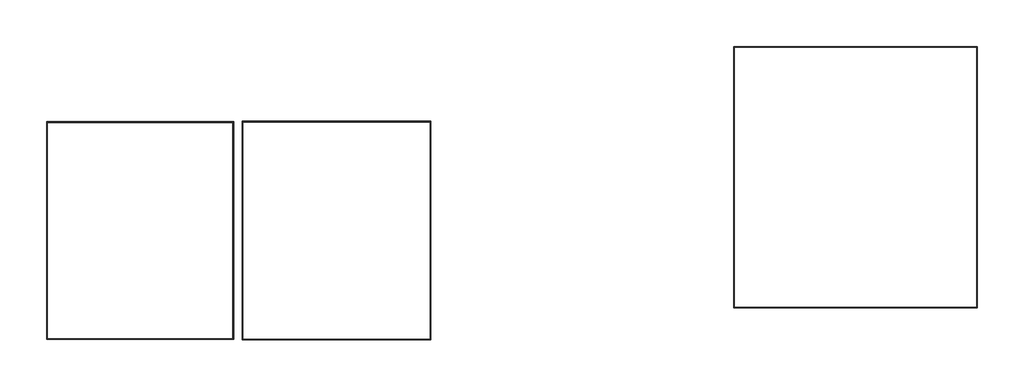
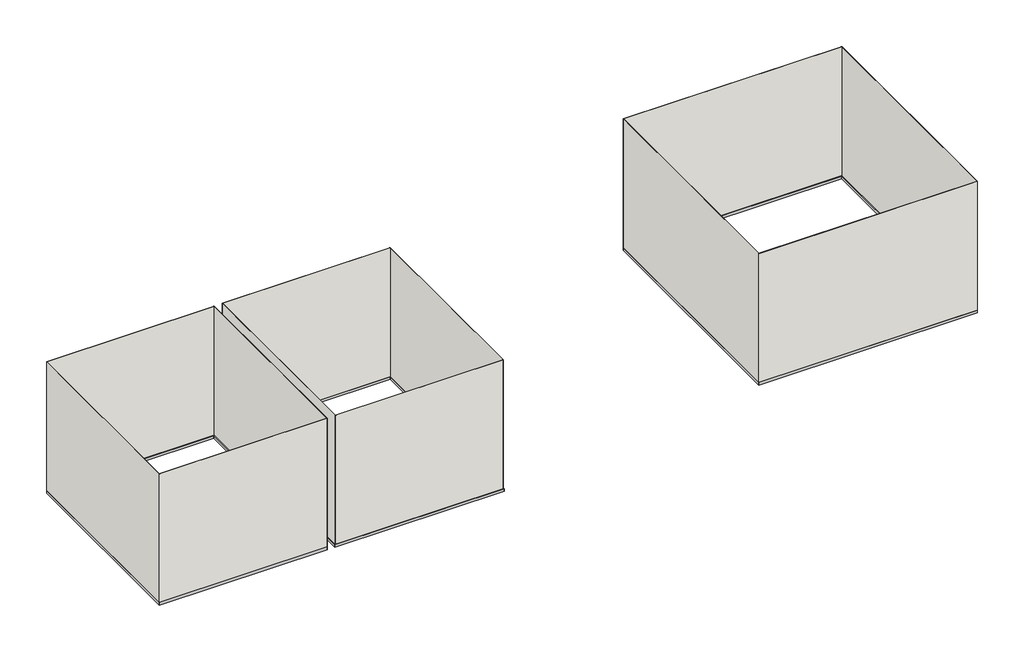
# Not in any storey: 12 proxies, 12 walls.
"""IFC4 building model written with IfcOpenShell, lengths in millimetres."""

from ifc_helpers import new_model, si_unit, frame, origin, place, context, project, spatial, polyline, outline, extrude, faceted_brep, element, save

model = new_model("IFC4")

# Units and contexts
model_context = context("Model", 3, world=origin())
ifc_project = project(units=[si_unit("LENGTHUNIT", "METRE", prefix="MILLI")], contexts=[model_context])

# Site, building
site = spatial("IfcSite", under=ifc_project)
building = spatial("IfcBuilding", under=site)

# Proxies
placement = place(None, origin())
element("IfcBuildingElementProxy", 1, Name="Wall Sweeps", at=placement, inside=building, context=model_context, shape_type="SweptSolid", body=[
    extrude(outline(polyline([(6040.0722622, 436.7286004), (6028.0722622, 448.7286004), (9910.0722622, 448.7286004), (9898.0722622, 436.7286004), (6040.0722622, 436.7286004)])), frame((0.0, 0.0, 12090.0), z_axis=(0.0, 0.0, 1.0), x_axis=(1.0, 0.0, 0.0)), (0.0, 0.0, 1.0), 50.0),
])
element("IfcBuildingElementProxy", 2, Name="Wall Sweeps", at=placement, inside=building, context=model_context, shape_type="Brep", body=[
    faceted_brep([(9898.0722622, 436.7286004, 12090.0), (9898.0722622, 436.7286004, 12140.0), (9910.0722622, 448.7286004, 12140.0), (9910.0722622, 448.7286004, 12090.0), (9898.0722622, -3708.7713618, 12090.0), (9910.0722622, -3720.7713618, 12090.0), (9910.0722622, -3720.7713618, 12140.0), (9898.0722622, -3708.7713618, 12140.0), (9910.0722622, 446.7286004, 12140.0)], [[[0, 1, 2, 3]], [[4, 5, 6, 7]], [[1, 0, 4, 7]], [[2, 1, 7, 6, 8]], [[3, 2, 8, 6, 5]], [[0, 3, 5, 4]]]),
])
element("IfcBuildingElementProxy", 3, Name="Wall Sweeps", at=placement, inside=building, context=model_context, shape_type="Brep", body=[
    faceted_brep([(9898.0722622, -3708.7713618, 12090.0), (9898.0722622, -3708.7713618, 12140.0), (9910.0722622, -3720.7713618, 12140.0), (9910.0722622, -3720.7713618, 12090.0), (6040.0722622, -3708.7713618, 12090.0), (6028.0722622, -3720.7713618, 12090.0), (6028.0722622, -3720.7713618, 12140.0), (6040.0722622, -3708.7713618, 12140.0), (9908.0722622, -3720.7713618, 12140.0)], [[[0, 1, 2, 3]], [[4, 5, 6, 7]], [[1, 0, 4, 7]], [[2, 1, 7, 6, 8]], [[3, 2, 8, 6, 5]], [[0, 3, 5, 4]]]),
])
element("IfcBuildingElementProxy", 4, Name="Wall Sweeps", at=placement, inside=building, context=model_context, shape_type="Brep", body=[
    faceted_brep([(6040.0722622, -3708.7713618, 12090.0), (6040.0722622, -3708.7713618, 12140.0), (6028.0722622, -3720.7713618, 12140.0), (6028.0722622, -3720.7713618, 12090.0), (6040.0722622, 436.7286004, 12090.0), (6028.0722622, 448.7286004, 12090.0), (6028.0722622, 448.7286004, 12140.0), (6040.0722622, 436.7286004, 12140.0), (6028.0722622, 446.7286004, 12140.0), (6028.0722622, -3718.7713618, 12140.0)], [[[0, 1, 2, 3]], [[4, 5, 6, 7]], [[1, 0, 4, 7]], [[2, 1, 7, 6, 8, 9]], [[3, 2, 9, 8, 6, 5]], [[0, 3, 5, 4]]]),
])
element("IfcBuildingElementProxy", 5, Name="Wall Sweeps", at=placement, inside=building, context=model_context, shape_type="SweptSolid", body=[
    extrude(outline(polyline([(-1799.4277378, -4230.7713618), (-1787.4277378, -4218.7713618), (1195.5722622, -4218.7713618), (1207.5722622, -4230.7713618), (-1799.4277378, -4230.7713618)])), frame((0.0, 0.0, 12090.0), z_axis=(0.0, 0.0, 1.0), x_axis=(1.0, 0.0, 0.0)), (0.0, 0.0, 1.0), 50.0),
])
element("IfcBuildingElementProxy", 6, Name="Wall Sweeps", at=placement, inside=building, context=model_context, shape_type="SweptSolid", body=[
    extrude(outline(polyline([(1207.5722622, -4230.7713618), (1195.5722622, -4218.7713618), (1195.5722622, -753.2713618), (1207.5722622, -741.2713618), (1207.5722622, -4230.7713618)])), frame((0.0, 0.0, 12090.0), z_axis=(0.0, 0.0, 1.0), x_axis=(1.0, 0.0, 0.0)), (0.0, 0.0, 1.0), 50.0),
])
element("IfcBuildingElementProxy", 7, Name="Wall Sweeps", at=placement, inside=building, context=model_context, shape_type="SweptSolid", body=[
    extrude(outline(polyline([(1207.5722622, -741.2713618), (1195.5722622, -753.2713618), (-1787.4277378, -753.2713618), (-1799.4277378, -741.2713618), (1207.5722622, -741.2713618)])), frame((0.0, 0.0, 12090.0), z_axis=(0.0, 0.0, 1.0), x_axis=(1.0, 0.0, 0.0)), (0.0, 0.0, 1.0), 50.0),
])
element("IfcBuildingElementProxy", 8, Name="Wall Sweeps", at=placement, inside=building, context=model_context, shape_type="SweptSolid", body=[
    extrude(outline(polyline([(-1799.4277378, -741.2713618), (-1787.4277378, -753.2713618), (-1787.4277378, -4218.7713618), (-1799.4277378, -4230.7713618), (-1799.4277378, -741.2713618)])), frame((0.0, 0.0, 12090.0), z_axis=(0.0, 0.0, 1.0), x_axis=(1.0, 0.0, 0.0)), (0.0, 0.0, 1.0), 50.0),
])
element("IfcBuildingElementProxy", 9, Name="Wall Sweeps", at=placement, inside=building, context=model_context, shape_type="SweptSolid", body=[
    extrude(outline(polyline([(-4899.9277378, -763.2713996), (-4911.9277378, -751.2713996), (-1932.4277378, -751.2713996), (-1944.4277378, -763.2713996), (-4899.9277378, -763.2713996)])), frame((0.0, 0.0, 12090.0), z_axis=(0.0, 0.0, 1.0), x_axis=(1.0, 0.0, 0.0)), (0.0, 0.0, 1.0), 50.0),
])
element("IfcBuildingElementProxy", 10, Name="Wall Sweeps", at=placement, inside=building, context=model_context, shape_type="Brep", body=[
    faceted_brep([(-1944.4277378, -763.2713996, 12090.0), (-1944.4277378, -763.2713996, 12140.0), (-1932.4277378, -751.2713996, 12140.0), (-1932.4277378, -751.2713996, 12090.0), (-1944.4277378, -4208.7713618, 12090.0), (-1932.4277378, -4220.7713618, 12090.0), (-1932.4277378, -4220.7713618, 12140.0), (-1944.4277378, -4208.7713618, 12140.0), (-1932.4277378, -753.2713996, 12140.0)], [[[0, 1, 2, 3]], [[4, 5, 6, 7]], [[1, 0, 4, 7]], [[2, 1, 7, 6, 8]], [[3, 2, 8, 6, 5]], [[0, 3, 5, 4]]]),
])
element("IfcBuildingElementProxy", 11, Name="Wall Sweeps", at=placement, inside=building, context=model_context, shape_type="Brep", body=[
    faceted_brep([(-1944.4277378, -4208.7713618, 12090.0), (-1944.4277378, -4208.7713618, 12140.0), (-1932.4277378, -4220.7713618, 12140.0), (-1932.4277378, -4220.7713618, 12090.0), (-4899.9277378, -4208.7713618, 12090.0), (-4911.9277378, -4220.7713618, 12090.0), (-4911.9277378, -4220.7713618, 12140.0), (-4899.9277378, -4208.7713618, 12140.0), (-1934.4277378, -4220.7713618, 12140.0)], [[[0, 1, 2, 3]], [[4, 5, 6, 7]], [[1, 0, 4, 7]], [[2, 1, 7, 6, 8]], [[3, 2, 8, 6, 5]], [[0, 3, 5, 4]]]),
])
element("IfcBuildingElementProxy", 12, Name="Wall Sweeps", at=placement, inside=building, context=model_context, shape_type="Brep", body=[
    faceted_brep([(-4899.9277378, -4208.7713618, 12090.0), (-4899.9277378, -4208.7713618, 12140.0), (-4911.9277378, -4220.7713618, 12140.0), (-4911.9277378, -4220.7713618, 12090.0), (-4899.9277378, -763.2713996, 12090.0), (-4911.9277378, -751.2713996, 12090.0), (-4911.9277378, -751.2713996, 12140.0), (-4899.9277378, -763.2713996, 12140.0), (-4911.9277378, -753.2713996, 12140.0), (-4911.9277378, -4218.7713618, 12140.0)], [[[0, 1, 2, 3]], [[4, 5, 6, 7]], [[1, 0, 4, 7]], [[2, 1, 7, 6, 8, 9]], [[3, 2, 9, 8, 6, 5]], [[0, 3, 5, 4]]]),
])

# Walls
element("IfcWall", 13, ObjectType="W_D=벽지/거실+걸레받이#", at=placement, inside=building, context=model_context, shape_type="Brep", body=[
    faceted_brep([(9910.0722622, 446.7286004, 14560.0), (9908.0722622, 446.7286004, 14560.0), (6030.0722622, 446.7286004, 14560.0), (6028.0722622, 446.7286004, 14560.0), (6028.0722622, 446.7286004, 12140.0), (6030.0722622, 446.7286004, 12140.0), (9908.0722622, 446.7286004, 12140.0), (9910.0722622, 446.7286004, 12140.0), (6028.0722622, 448.7286004, 14560.0), (9910.0722622, 448.7286004, 14560.0), (9910.0722622, 448.7286004, 12140.0), (6028.0722622, 448.7286004, 12140.0)], [[[0, 1, 2, 3, 4, 5, 6, 7]], [[8, 9, 10, 11]], [[3, 2, 1, 0, 9, 8]], [[9, 0, 7, 10]], [[3, 8, 11, 4]], [[7, 6, 5, 4, 11, 10]]]),
])
element("IfcWall", 14, ObjectType="W_D=벽지/거실+걸레받이#", at=placement, inside=building, context=model_context, shape_type="Brep", body=[
    faceted_brep([(9908.0722622, -3720.7713618, 14560.0), (9908.0722622, -3718.7713618, 14560.0), (9908.0722622, 446.7286004, 14560.0), (9908.0722622, 446.7286004, 12140.0), (9908.0722622, -3718.7713618, 12140.0), (9908.0722622, -3720.7713618, 12140.0), (9910.0722622, 446.7286004, 14560.0), (9910.0722622, -3720.7713618, 14560.0), (9910.0722622, -3720.7713618, 12140.0), (9910.0722622, 446.7286004, 12140.0)], [[[0, 1, 2, 3, 4, 5]], [[6, 7, 8, 9]], [[2, 1, 0, 7, 6]], [[7, 0, 5, 8]], [[2, 6, 9, 3]], [[5, 4, 3, 9, 8]]]),
])
element("IfcWall", 15, ObjectType="W_D=벽지/거실+걸레받이#", at=placement, inside=building, context=model_context, shape_type="Brep", body=[
    faceted_brep([(6028.0722622, -3718.7713618, 14560.0), (6030.0722622, -3718.7713618, 14560.0), (9908.0722622, -3718.7713618, 14560.0), (9908.0722622, -3718.7713618, 12140.0), (6030.0722622, -3718.7713618, 12140.0), (6028.0722622, -3718.7713618, 12140.0), (9908.0722622, -3720.7713618, 14560.0), (6028.0722622, -3720.7713618, 14560.0), (6028.0722622, -3720.7713618, 12140.0), (9908.0722622, -3720.7713618, 12140.0)], [[[0, 1, 2, 3, 4, 5]], [[6, 7, 8, 9]], [[2, 1, 0, 7, 6]], [[7, 0, 5, 8]], [[2, 6, 9, 3]], [[5, 4, 3, 9, 8]]]),
])
element("IfcWall", 16, ObjectType="W_D=벽지/거실+걸레받이#", at=placement, inside=building, context=model_context, shape_type="SweptSolid", body=[
    extrude(outline(polyline([(6030.0722622, 446.7286004), (6030.0722622, -3718.7713618), (6028.0722622, -3718.7713618), (6028.0722622, 446.7286004), (6030.0722622, 446.7286004)])), frame((0.0, 0.0, 12140.0), z_axis=(0.0, 0.0, 1.0), x_axis=(1.0, 0.0, 0.0)), (0.0, 0.0, 1.0), 2420.0),
])
element("IfcWall", 17, ObjectType="W_D=벽지/거실+걸레받이#", at=placement, inside=building, context=model_context, shape_type="Brep", body=[
    faceted_brep([(1197.5722622, -4220.7713618, 14560.0), (-1789.4277378, -4220.7713618, 14560.0), (-1789.4277378, -4220.7713618, 12140.0), (1197.5722622, -4220.7713618, 12140.0), (-1789.4277378, -4218.7713618, 14560.0), (-1787.4277378, -4218.7713618, 14560.0), (1195.5722622, -4218.7713618, 14560.0), (1197.5722622, -4218.7713618, 14560.0), (1197.5722622, -4218.7713618, 12140.0), (1195.5722622, -4218.7713618, 12140.0), (-1787.4277378, -4218.7713618, 12140.0), (-1789.4277378, -4218.7713618, 12140.0)], [[[0, 1, 2, 3]], [[4, 5, 6, 7, 8, 9, 10, 11]], [[1, 0, 7, 6, 5, 4]], [[7, 0, 3, 8]], [[1, 4, 11, 2]], [[3, 2, 11, 10, 9, 8]]]),
])
element("IfcWall", 18, ObjectType="W_D=벽지/거실+걸레받이#", at=placement, inside=building, context=model_context, shape_type="Brep", body=[
    faceted_brep([(1197.5722622, -751.2713618, 14560.0), (1197.5722622, -4218.7713618, 14560.0), (1197.5722622, -4218.7713618, 12140.0), (1197.5722622, -751.2713618, 12140.0), (1195.5722622, -4218.7713618, 14560.0), (1195.5722622, -753.2713618, 14560.0), (1195.5722622, -751.2713618, 14560.0), (1195.5722622, -751.2713618, 12140.0), (1195.5722622, -753.2713618, 12140.0), (1195.5722622, -4218.7713618, 12140.0)], [[[0, 1, 2, 3]], [[4, 5, 6, 7, 8, 9]], [[1, 0, 6, 5, 4]], [[6, 0, 3, 7]], [[1, 4, 9, 2]], [[3, 2, 9, 8, 7]]]),
])
element("IfcWall", 19, ObjectType="W_D=벽지/거실+걸레받이#", at=placement, inside=building, context=model_context, shape_type="Brep", body=[
    faceted_brep([(-1789.4277378, -751.2713618, 14560.0), (1195.5722622, -751.2713618, 14560.0), (1195.5722622, -751.2713618, 12140.0), (-1789.4277378, -751.2713618, 12140.0), (1195.5722622, -753.2713618, 14560.0), (-1787.4277378, -753.2713618, 14560.0), (-1789.4277378, -753.2713618, 14560.0), (-1789.4277378, -753.2713618, 12140.0), (-1787.4277378, -753.2713618, 12140.0), (1195.5722622, -753.2713618, 12140.0)], [[[0, 1, 2, 3]], [[4, 5, 6, 7, 8, 9]], [[1, 0, 6, 5, 4]], [[6, 0, 3, 7]], [[1, 4, 9, 2]], [[3, 2, 9, 8, 7]]]),
])
element("IfcWall", 20, ObjectType="W_D=벽지/거실+걸레받이#", at=placement, inside=building, context=model_context, shape_type="SweptSolid", body=[
    extrude(outline(polyline([(-1789.4277378, -4218.7713618), (-1789.4277378, -753.2713618), (-1787.4277378, -753.2713618), (-1787.4277378, -4218.7713618), (-1789.4277378, -4218.7713618)])), frame((0.0, 0.0, 12140.0), z_axis=(0.0, 0.0, 1.0), x_axis=(1.0, 0.0, 0.0)), (0.0, 0.0, 1.0), 2420.0),
])
element("IfcWall", 21, ObjectType="W_D=벽지/거실+걸레받이#", at=placement, inside=building, context=model_context, shape_type="Brep", body=[
    faceted_brep([(-1932.4277378, -753.2713996, 14560.0), (-1934.4277378, -753.2713996, 14560.0), (-4909.9277378, -753.2713996, 14560.0), (-4911.9277378, -753.2713996, 14560.0), (-4911.9277378, -753.2713996, 12140.0), (-4909.9277378, -753.2713996, 12140.0), (-1934.4277378, -753.2713996, 12140.0), (-1932.4277378, -753.2713996, 12140.0), (-4911.9277378, -751.2713996, 14560.0), (-1932.4277378, -751.2713996, 14560.0), (-1932.4277378, -751.2713996, 12140.0), (-4911.9277378, -751.2713996, 12140.0)], [[[0, 1, 2, 3, 4, 5, 6, 7]], [[8, 9, 10, 11]], [[3, 2, 1, 0, 9, 8]], [[9, 0, 7, 10]], [[3, 8, 11, 4]], [[7, 6, 5, 4, 11, 10]]]),
])
element("IfcWall", 22, ObjectType="W_D=벽지/거실+걸레받이#", at=placement, inside=building, context=model_context, shape_type="Brep", body=[
    faceted_brep([(-1934.4277378, -4220.7713618, 14560.0), (-1934.4277378, -4218.7713618, 14560.0), (-1934.4277378, -753.2713996, 14560.0), (-1934.4277378, -753.2713996, 12140.0), (-1934.4277378, -4218.7713618, 12140.0), (-1934.4277378, -4220.7713618, 12140.0), (-1932.4277378, -753.2713996, 14560.0), (-1932.4277378, -4220.7713618, 14560.0), (-1932.4277378, -4220.7713618, 12140.0), (-1932.4277378, -753.2713996, 12140.0)], [[[0, 1, 2, 3, 4, 5]], [[6, 7, 8, 9]], [[2, 1, 0, 7, 6]], [[7, 0, 5, 8]], [[2, 6, 9, 3]], [[5, 4, 3, 9, 8]]]),
])
element("IfcWall", 23, ObjectType="W_D=벽지/거실+걸레받이#", at=placement, inside=building, context=model_context, shape_type="Brep", body=[
    faceted_brep([(-4911.9277378, -4218.7713618, 14560.0), (-4909.9277378, -4218.7713618, 14560.0), (-1934.4277378, -4218.7713618, 14560.0), (-1934.4277378, -4218.7713618, 12140.0), (-4909.9277378, -4218.7713618, 12140.0), (-4911.9277378, -4218.7713618, 12140.0), (-1934.4277378, -4220.7713618, 14560.0), (-4911.9277378, -4220.7713618, 14560.0), (-4911.9277378, -4220.7713618, 12140.0), (-1934.4277378, -4220.7713618, 12140.0)], [[[0, 1, 2, 3, 4, 5]], [[6, 7, 8, 9]], [[2, 1, 0, 7, 6]], [[7, 0, 5, 8]], [[2, 6, 9, 3]], [[5, 4, 3, 9, 8]]]),
])
element("IfcWall", 24, ObjectType="W_D=벽지/거실+걸레받이#", at=placement, inside=building, context=model_context, shape_type="SweptSolid", body=[
    extrude(outline(polyline([(-4909.9277378, -753.2713996), (-4909.9277378, -4218.7713618), (-4911.9277378, -4218.7713618), (-4911.9277378, -753.2713996), (-4909.9277378, -753.2713996)])), frame((0.0, 0.0, 12140.0), z_axis=(0.0, 0.0, 1.0), x_axis=(1.0, 0.0, 0.0)), (0.0, 0.0, 1.0), 2420.0),
])

save(model, "model.ifc")

# Revit data of these elements
# Project information
#   Project Issue Date = "발행 날짜"
#   Project Status = "프로젝트 상태"
#   Client Name = "소유자"
#   Project Address = "주소를 여기에 입력"
#   Project Name = "프로젝트 이름"
#   Project Number = "프로젝트 번호"
#   DBIM_PRJINFO = "190232▤101▤01▤01▤▤1"
#   DBIM_ISSELECTEDHOSH = "N"
#   DBIM_STAIRS_OF_CARRIAGE = "<DBIM_STAIRS_OF_CARRIAGE>\n  <xs:schema id=\"DBIM_STAIRS_OF_CARRIAGE\" xmlns=\"\" xmlns:xs=\"http://www.w3.org/2001/XMLSchema\" xmlns:msdata=\"urn:schemas-microsoft-com:xml-msdata\">\n    <xs:element name=\"DBIM_STAIRS_OF_CARRIAGE\" msdata:IsDataSet=\"true\" msdata:UseCurrentLocale=\"true\">\n      <xs:complexType>\n        <xs:choice minOccurs=\"0\" maxOccurs=\"unbounded\">\n          <xs:element name=\"DBIM_STAIRS_OF_CARRIAGE\">\n            <xs:complexType>\n              <xs:sequence>\n                <xs:element name=\"Stairs\" type=\"xs:int\" minOccurs=\"0\" />\n                <xs:element name=\"Carriage\" type=\"xs:int\" minOccurs=\"0\" />\n              </xs:sequence>\n            </xs:complexType>\n          </xs:element>\n        </xs:choice>\n      </xs:complexType>\n    </xs:element>\n  </xs:schema>\n</DBIM_STAIRS_OF_CARRIAGE>"
#   DBIM_ITEMS_1 = "aygIAB+LCAAAAAAABADsvX2PHEWWN/r/le53KA0S2+4ms+ItMyI14yvZbYznETYWWNs8i0atzHqZXWkY9rnD/LHCSAYa5KHNGh7cQzNje80dM8azHm1jGp5Ga3+hzqzvcCPyrSszsrIyMyKzuk2ZUeOJaurEy4kT5+V3zvnF5X8bvfXbX/d+OTz9M0B+1rvkvjk6/TNGfvb//N//V6/3iwtv/f53o39+6zfD6BcATH7j8GAvuH8tOPgq+kX+q2fd341++fbozd/FA1NDPfFj/a0h/+8uQwxsywIW+Fk4Gn2b//DW5IPr/p0nwcf3e/53+4d7Oz/rnX/r/33z979xo//OgOnA6Z9dDbYO/BvX/O0f8UV0tfcG/tXPev25ZBnCAGXIBn/a8+9dn3yw5e89DK7vViMJD/duBx/duNqDFYhCax1fEbs2RfTprcn7P/aD7fv+Xx8FT3eD958c7r2Xoz1F+R1k4ndXrSNiv+jnt/oX6+5vBrm9T4Zm7H29zX119Lvf/+bt9FdwMvKP7m9+Pwr/f38u5WT76+5xjjbM0YYVaKenMHePc8T48NFoQhCamcPI7/0vXn3rrTfD6/JP//RPQPyBVnJrgh+/4eeOf3Y04Sv/9q+j8JeHrg2GY+gYwB5aBmHewGAuRsbYQXzrhsMhBMzgX2Yjz2bJ950/Pbnxqb/1aHL3+uTGh/3o61eCg+8P97b4/gV3bgRfbgU/PAzuPupfweDUGr9Y/oPr/l++ee5oDoV3t/z+whxPZ2YRiYZ4Mv3MZO4+4rOYfQzrb/32bfdffvu7jX95+59/t/LrzQuvbV66+MLz/+v3b7398+hbo7+/cH7zTDwcfH87+OC9qWFwapoh5i6DzFwG/+bJzi6ffrySFw6/3eP/ajb76MuaTBNiAtfh69PTTA+xH9x54u/l5dbUlDilLBlZdoSjv/zt7952fzuIOHHsjOzxYMxZD3J2JEMXGw5FtjEeD4AHLduDyBWcOCI2wj/LrkEWRPPEESy9mLo4Inevs187/XX8RYv/0wIiEJjEoaSIUPLREbFEXEQf5E97zpYQjWzWeO2Zb5u5QFB5aSkrl7JrXt4n+1dlV2VpHI0m/H0kd/tC8BaIYTgiljfE2KAAuFwMM8vwLAgM5DmWh4euC2DI/BZmBCRieGPz3Gn/8dPgQSL11g6/PeCahb/35+DOvoKoFTv2Uu7yT31z//D7vwfv77124cUXr8ze1Y3N9ZerChuC4Gsgq5pNr0toLZP3Hvlfl8icjc3LZyqTcyDfSpmc/8OXfHmcK2O6dahpFnFsrCbi0iMsP54815vEppLmEQ9WvW7JYZbvXV63M7mqBvKk09HKtOOTbY925buucPgOWMThI5PC/CbEY60ePTGZjSSuS0dbPfpatDs5erSIowcmP7r8LiSDrR4+MPl/SGTS8Wirh1+LduPDdz0wtNnQNTCXJwYZYGK4tgUMF7DBYDAGNsPi8CFAFl3U4TsFZ++0f/TEwnkNKxls+eArU+7g2NnAWcyxW0SSfMlgqwcPTYTl9zYdbfXoa9Fu//Cxhb3FHD6meXdaPNbynWfYKXhp4tGWb30N2uomXXUBYOPUv33u1c2Nc9ysC7545G//JzdG/EcHsTGCn+s5AKwiRMEqX72KI40gTjbjHN57Otk9CP7yJLi9Fbz/KPjhfn9yc184io9c1bcnNx/N3vEVMfM1/uPCKqrsY+J/MMqYmRvn+s//5u2fRx7Zyc0/THZ3nv/12z9PtmA2fVidJs254/kWBw/uCP9/8MfPNFHA7VJgEL2e2Tf/5lbwx33/qzvxTgV/eqiFDi6kE3x8f/LRvcknTzRTYwg4Gbb86FP/vSfB3TBQ8uCaprOB+bOZbF+bezakVWvfgaoOzfhKV7yeOcm4AkxnDZmITn0Yi0fLJDW0seRCl5xTnbjKPGJUjuy0SawshqCXWHy/OyKGuyQW3fHOzqzsUhCJWN4maMHTW10toE4aGN+4tHmZ63Gng+3bQvZ+eJs/2P3okQy+PPB/uPZcDxKhF/AVKygGmIDcy7X+yqV/WPcf7gePd7k2UBZFXeFz3FjjP4SEWX0HmOjdqhExQZY0JCuo1qFjN6RT9YUJJTGarVz9wB+yLf9ve5MPrvf9/zoI7n6taXVc8p4BgE0T5iwDTUJfhyakfUbixxq9ECtTK+j8Cwic50pm8MF7p3Qsnv/D6GzNsheplm/47+8HB1/9qho3nVpFValbfPtz1K/vBlvfTv59N7hzMPn4oDLFIv7V/eSrxjCTy1rzSuaffsEha4JDxO/wX5HMI2pLB1A+KVI6qYil5bgDlaMOtB5du5SuzpclveQdLzO9490sM73Ole/pTOaa+jRVLPkDN/2nhpqZXPSat7lsdgWsD01gWdMzZIuN+6KjuO96O3Hf8BrB6i9kxuPyUuXw6zK6XDu6XEbNyVu0N7m9vOfv3Zp8sCNO7t7OnJM7324om98b9ZeuTI+PeE8GcEBoy/iNcLAGcqS+b5WYSIqjxmOt+lYdkzAsefTT0VZ9q9poO3NO+nyRS58RJsnucEy78caltQcgNtyR4HqEqMGcETAGeERtLqEpHg0F17uIwVEirtdfPB08vs2vIZcBSqAcBFFOruztBnc/nWxfC7buBz+WiK/1PCCvRJ7gvLBMJ98PdrYmN25wRbqKyKxD00E5iZnSnBKaCfEaJHVLMuVYTXyEpQuQrpZj47wgSwYrXyxcLlDaIxwfbUuENWhgjLgYA8fAgFKDvzTIcFw8NFxoWwBansWcEADtMeGlTa702dPBf9+ffPzE39sJPr6/Mtl5OLnxaX8DWuDUZvS6P9frXYBEwRvDmcWCMHsrOM0PP41olmzp2c0uVaMVTm9jlf84V8NU1yZlUuovn1oTfz8X/b07Xa3Z8jUJvEqr1y0ER8pCMOLrcv6VwWl5+ywa0qVS5c5RjpBAa1UgomRLFpiA1JnIHFE880wLpyQ2gf+emFn0d9l/wxgDR39gDXfDPFWwuz2b84p0vmfq784Ye2MIRo5B3fHYINjjSqUHmEE9hIDjOoAMrPDG2cNRGge48Opp/297/q2HsVhSUicxyov+6a8ujeleeDX/xFQSMtWXPFQWMvHqyleQtySwKVmM4ZDuw2cD5NrIdY0hJEODjBkzPGo7hu261pDLW2oxGu6ER4ewGtx/M3h6y9+6vkT9Pzt+mQbGTA2wqa18xRqCTa0ipLHVBdIY2wVA13i0baSxHtrz3COFpKmEd0wGu8e6Uvsnx3XEKUBahoNt85wOyo04jiFWwHLR6CJ9cvbRW3p2mTr3k3hEmwQ3amB0RgvB7iMTOpK3PRlsOVnL4fdYim5Egy2nammh3CjAgAguSBkIB7WbBtzc88h4aFi2DQwCwdBwxoAYDrOHWITJXXsU+iPJeIQTcfbihoCGTT4+iEoJrFxxTm1ePuc/uH74/SN+P5TkmU3ynropSmUx+Bc3Nl87s4rW+L+vtHkJ+YumfAnjRVZejPTkIQj5p8AEeYCHyBiX/YLKbELgaGzh8chw+U+DDPkWMYfyR5AiMoCAjSBzQjYRm5i+ejkugeiUImu83ow12rVtsEWVE2jjpc1ZgpxXhhHLuxDSUe0uJNuCnAU8Yzyy+Ia4nm0wjBzDcyFyx86AUnssNgRib4inopFp2DB7+FlfTeXvHnqZUgyZ2f6iL6rSJP9HrlBDshVq0LJCzQyX+LJCTaHmdHwr1Cg6V05ehRro2GxGhZrwo6IKNeKDZ6FCTfEC269QE+1flV1Vf2xsa4QxHFBjOASc+UcDYHj8ETCo4zJIBqMRGIJQDLsMjJqK4aXwPV7CV7NUxIOflFQU2HmriEz0gSwwxPCJl4ezFrfAVCowom4qki6dPty7xu3izXO/f/PNf+sSkJdFqJ+/tLmxyn+0DNegpA3M2uylyBF3exWaVHr9TdCCVbyE0y89zifS41znQluLgNPza8wIzGub6WirgHpgIlYQvYsGW47e2YWLrrXmhtE7LZQbeLs5EcsqCBzGo92XRKMLyR+hJoSWFG9IR1tleGQ6chnGZLBVhrdNm0ou7GSwVYbXRLlReIdQqQpcMrhIDWVZ6PU46g66n/OFAGKwCaQctXisVflimRZjkmhLR1uVMLVod/KwLQSBh/mC5aO3ZGiO5qNnJhdqTo5wMtjqwdeg3MWxM8ViT02VaFJU7pF0Ue6Rr1uuexANtlzssTLlDrCPA7Kggwe4wHqKBlu2niCwZUMiGmzZeqpMucuKTp5LKxR6RFOFHtEzU+gR4RqFHtFs+stCj8tCjxXP5hgWeqT0mSn0GF7oknPSV4ZoWehxWehx7pktCz0uCz1O01kWelwWejwWhR6pIjh9WehxWeix5WUuCz22XuhxmfH/jIR/WoWOtBxqWkhPwWXG/zOY8V8n3LGQZobABEWYIdAFZgg6BcidaLBtr7cOyk04jtv6Bcwejy6rcEbbtKzCqac1biuI5vwCcizucMmdDyHHY+3W4FQn26gCZ0Wyy/qby/qby/qbndbfZMNF1N/EYb5GHi+2rL8pNiGpJRn+XZoc46a9PsXvhJbcbLZNyyqbbVbZpAQq9iBqWGUTmVJ6QTym+/gR8Gxk2ciwbObxvWBDg/FbYHgjLgQJHDh4hEJLYYzhVJWUKEGQv0SbwzBHsHcFgZJSGYQ6o7EzNEYDvuuEWdBwEcAGg0MytsAQO3AQbviYuMOZpTJ6x62wB+EqV9PCHiidVZyeXLDIOnU93BkJ5dG3z0oot7XW9cDzUsujyUip5VK0Yvqp/emmlpc6pY9tXQ+imnyXsFLbHKGprgc1+ZyL63rEH8l1PaIPTnwe+8wFtl3XI9m/Kruq/kRS6o4GyHUMdzAYGoTYnuGNrZEB+DNBwcAekyEUzO8M6SBNmX7p4mkBGH30RJhNd7/uT77c4f9Sc6vhf8wZpCmBezsxAQ24QIzOACdr+YUiJdi6c/jdPf+7ff/z27PJvHRx88Krq/znP77auaXdhLYmM3cmab3SlULlXKiYi0rYRGPQPGalSrsmmdMIid4DUt4hMxlmGp2K3Uxijq2ocRJdRuKtES2IxEda0QnOwMTFHsdEfW0hBG+XOfjmaZltZ2BSqNzVq1mXQKugS6BVLwMTNyngC225dnA6WstPZbdJu4PYNFUt09c0A5M6sjOVymViNR894+zF2V2Ss/Foq0dfi/YyRLwMESvda6jeo6x+iJiaNpSipslgm0FiPYQbhIlrEO7UUPWGlQLFkebx3MmIEytrbSc/TqykRv7U4sQUKePumsSJuQor92iwNGo2JzROLDYhCYCGf5cw6BjWcJrOVcJOaJy42TZ1mKyHwWBcI1kPR0n8y2S9cjrPeLLeei5ZD5uIvo5MECbrFT5cy6y8drPyKEbHIytPsMKaYIXirDxoEoamOtHWQFw1TdETM5KcE+iZS9FTXWZ6s7tZpnqKXspp8pMPRR3XzrPypidUwPrIhLiFpjkWdAl/6IHBRjYxCKbQ8Lg4MChw+TvPLwyw7PClt6E1mEKERZLUf//24d7WygXItS+l3km24KCsQbd3WyT0bV+PaLwhSEQp23lRrQ4RqyEnVVtrJQstX4F0OfMAsXBkcSUahiP3CB7GTc/JB9eCO09C0+/jg+DPt9aigeDuI/8vN/wftrjewrVAFcyRA9dliz9PtswJW9WpBxzi5MsYJZRSI1cPIQfmCBXuWhmtC+0yu2p/iuTQSjdL8oxjhonsGY9Hqz6DySkugnR8rqXHliONpBuO2rjhgPDD9/hpD8ZjaBDLBobncl4gEI6gjUbIi4O9I8sby/jf2EOohP+VEjymv7oF/G+dJSvye7q6WsIdQlNCN4VDixPvI88t6AahN9L/zHaDOPF4gjJqx7z/8NBRhEw17QaBKcoHfpLBGuDIRtUEisrYwpplbBtEz/nyLEDl9Op4tNXouTbajfpBYItJUJV0VHvGzvHIfcgW66mV+3DU1PQvT/y9h1O5D4U3f5YcZ3kDMYpd+t/tH+7tlBnfV/3tfX/7x8sXJ7ufBXd2ubgPfrh9tfeOqP3I31mad6zNcuet5yfAzdPJ+z8KiS4Kxj7l3/zkcO+90qlMdnb9H64dHhxw4Xz1HWzaYgaiT7Jtvdtb6131P/rf4SfApNYqXuM6IB++Gtvan+3yd+vqO5DLFfFf0HezvsgiSVoo/mYKIFZgmtbdSum2RJ9Iyi3NuZZmOlfW505K/6ZK5vfUV64dfc1a+l/JLiRi0mk/JYDZo5LPpVkmkNc0E2gzuo1Rale0g8uUoJOSEmRBOx+HLw0tTM2o7YwgWzHMfsIygrAJiI1IEaHkIylhJv7gxGcEzVxgjYyghJNL2VXOvY/2r8quqmtgZADAcEQ9w6NCHI/xkCtIQ640eQPijr0xdcZeaH0QboqUekW79n9moz6tekDLSemGMyoWbiv2S8pLkPiOUNkPH44peSX1Ee4QVTii1JkZDkKWajQI8q8oiwbRMBjEZdECg0EMu8rBoGid9fyFZl70hSMLFHsAH4m94Itbwv20fV20Zfg8BAJ9dL/P5YcKPwAo4Q6LyBw5vTg9HSEaQfhithHEzPXVoFeFDSunZQ2hrVrHMtneOrESZLK8wysaqvryJ1vbAtHGqTI1Nn2o2IWz0aaLJq9yy7Z0tM2tr0W6kwNQDdY0OQAoqoLLyejJaJsHUIt04wOoLPUtgBZzAwiSaokng+3yf2XCHWw+1xwWsvmA2YVVZO06ZWSbbX8N0urKz7IYz9LzdjyK8VR/EbFqhssJc71BZCIbQLuwGk/ymVyOJ/7kxHvfZi+x7YI86Q5W2tgOcStgRI+E8aW4bN3mubBmXYf5y1no7/lLmxur/EeT9Lbql99iqr6IwhTf2UvJo5cRV4VWgcnsPDci/kZDOWmicTWDqtUFR2OqXMhCbUuAiZG1KqKfcnlPG1CdJR4ql1wE6jUudWwKNrGcygZoG6pcJzUvq19UGw5zcqChCUAI0/RFQmjq+CJrMBsk0sizaAF3UKcTIKZg1V7mFpbTecZzC6nUCBDT1wVEI2wEGCGQNKzyJ59bWEPiWYrVR/R1/EvROsUd/6waid7NO/5huRUefubSCVWXmV7mbpapo+NfzFxyOiEx6/iGtfX4O5pPIbMzgbyY+tOG4basOvXMVZ2qIfdd1QBBk6pTUDS3dCR89tFwm5Wn9BFvUH2qJvFlMlm7yWRD5e6SjZLJkEkLPHO0BelevXAsHk7h4rgBx6VS5NxfueIo4YSwTfLSd+rbtUPUapjCRFn2xUurhxQDJnas/Pkng9oRQgQiyxq7BrOYbZDBGBuO4zGDCV2Ka1Mu3y7BAGMEBqPZDKCvdLA+bigNADXLJ8wRbCB86rCfciZrI/ZDJnGktKxkUCkPTt49yeAATBJ80djiBN+yYvYscse/Ynb12yZQ54q3rUnqp4i4yFet7aLJlkmk0vTxWKspn5XpPiMpl3gEGqdc4rQx6GR363D/WlG7KS6mPMjFowFHlBgEhBOBruGNLITZAFpDB4Xs7dpHj/f5WfDevVv+tlK/EwBxNaBtSKnscZBQFqVEa8KK51LvFDQTLYB2toC5uBnNuWSuaqwy4ao53CIJVouLRlmNiUerw9ywbMO3wix68DTxAosIJR9JUJNmm1Lq1l0QnGbmEiU0jY6aa86I20yeMbItbjjZA8LFLtcnB3joOZggOrRD2ctvgj04ArRswtORPPdv3fJv3ReFu4PteyIz5u7XUQbvSrHQvILA6gbf91Nr/t7DyUff+w/+oKhzAkgunkUZtF52Zm/kZvarPiNnXnDwmRfOvrD+wrnSK3mpeh1wbNF8Un4UEk6o96ZXPFvliJLH1yY3/96uQFNVFJN9n7d7MngfyNhlBGrEY5KdrrKDRdTXgFThCpiWPINOsbu0cfr8ErF7vBC7ui8q/UlBaYFJgFXc1zL5SH4Xow9OPI529gL1i6bRCA0dMhgbXAhxo4uCscFsyzWGjDoMjRyCx2F2rTWgbiqaQvzq5vorl9Y3r4hsUS38PbuV8TKA+2wHcOtwSSsA2jlhTGQiCqw8lCMdbTN8q4t0g+BtLdJdNg8aOHYqiF7dPP/aOYHB/OKRv/2fnE/9RwcxBjNS/5/riSrNq4ivX0U/IgjkGghNAwhDZF3f3/4m+GI/whFyrXNflOD6055/7/rkgy2u+k9ullQhXOEr2VjjP+pA7iCBMOtm55uRWX3/+d+8/fPJzT9Mdnee//XbP59NvzLIEDJuA8KMCLwlDLwJp3pzS9h4X93JTKE05F2DLIZZZ1xELTQn700+edIKTVJM8/E+l7ytEKT55yUhGNwpEbqVCVgI5qX8V3uiaN38Ik0hg65GDAoKSsHOomjnKR7uf+b/7UN+VyrT6lfHoK5L64sL4iX3sLAg3qx7mL+Jut8y1VrWiVSqKFRkPB5c4+JcRgfaZhaHB2pEUhKZVMKr+iCSiTDqiFgkgjoiRrokRkt1Iq3EEhlUWdAUsO1qyLZALlJtOjjDutUrmqWSqoZQKptZX4a3OjbLlF+sUZkkEWyVxdbsuy7XhcRmpn8NaEG5q+FeZuMy9/Jcd3KuU8FKFF7qT7586N/8UrO3GZZ4m9txLtvMyiEPyjsz/GS82EMdXuz8SzLfiw1NJCN8UPVM7vRAu6ar4DsXhApc59BsA9BXwypk05iA7dv+w12u0EbW2MoVvlhFBznK3Yf1i0K0fF3eeqVr9zeCRO8ku/Zye+oFI1ApYx83L7fDVVir2MsdfVTg5Q4/qOPljtji2Hm5Zy1wWa9BX72GOndPtYCTeh4+E7UJYEFtAkYzurO+6mLV28qOPFUl4yTsjxb/LJpKrYn04gz+d7L1bSk4hCvzitVaAbQunsWyej49jTfSaZQjQaT8lhav4EC9gF208PIVyOVbpXYI8Zh2LhqNkTseuMZwRAYGgZZjsDEcGIy5DvUw9lyHhAkaY5uRUi6awTsErFI13lEyfTK3WWaXORxLyjm2Hi3drKks/YpMjoI1SMxpSUAhWATTmXMp8mF+jZS7zFtCw0bXAilfi3ATC/B1JQzaJXsO1XFsloxjm8ci/EmWIWS4eRF0lQ1QL7l8DDZAi/qBm98QbQ7CBb4icy5pdc9k+5dWuUJc0zeFQrlifThW600phb2qUdbwpsDR2MLjkeHyn/wcuHnDHIoNlyIygICNIHPEOYQG0KxcWIhUs6Ff7zAbuk6jBGV1Jl7anCVI8pI6mOQ5IB1dmN+DAFEELjqiF+WE6M1IjJx/7Zz/4LooQvfXR0psAS/k4DQRdia4W8oTL25svnZmFa3xf1+pnh3NRUS29lfcpe+TB/4ne3PaxjSj2Djpu4ScbvZXLICVHmHlxUgXwbLYquhfh5gcSsBOnS6l8Qkfh6nMzVHXPJVnrRilh/N1QZp+kZWt+7ssGdOkZIxNlWuzNikZQ0yWh3ZEQ89mXvWY4JmsOi+vOq3m4H+3H3y1p9LQFjAkJR8f4VcfBtdLoxQ51EgZRC9b77MSRC/bXjXCph9+d291/VVRKrQnSk0+eK/n3/wyuPNEQCL42CE3sz66cbX3DjIReXcV9dbCvzLNPWrTXSvdmnr4qTIYUHmhRQ1bI8PACX+RxMcSdMgxswir8iaylVM3LNE34OiyHT5+6v/HH6KF8SvH9VHT6sPLp9aiAqOXV9JObGq2CqJ21mLPEdaSaGHJfcOq9kmtQ8WBuWKsk0+eTLb3+v/jlV9eKim60nL6BgXKZUniQypdQI6DsUm4hphj3WSweg3M+hkUegjHR9kS4Q4zyBxvaE/XHpKvb6YA0eWVCxCIrtDh/Tungt5hSMjo6g9bxoivXIZIkDmTM2vDb598eEN0hry1pYUMxAzlLje+2MtR6hU2oW9I0IISrL6qzNrYfKm60CIkT2brwL/zxP+vJ5Uorb8sKs/CqiXOGwvJWmtaF7XPVDISrkYI1h4/1+DBdf6AX+1Jpdq0q1uyRnGkQBTQ12p0DMe2rQgCS+57OfNLtrcDCroJRoNVsVaJCOiccioVuqeciIfy+yKplRA5ko8jHa1MO5YZVaRC4dpX+WfS+kHNDZjzRLe6AbGAqSs+WmGEIvOkgihpPpfGgdXqLhBsq6ZpNZJGkK9XqpscjbUqi9TpNpNEGug2kkNEFOyTKlSnox3IoXCVhWII1lt+Eymka/l6pJAOJtAjgyrPpP3OqurZLU31IVokhmkX+pA65ab6kAbKjeQQNG0bFsR84tFO9CE6Ux8Sn0zji2uA7xqJJV27oUs50sEVupSjynNRd+1gDziQAM8YOCOuJQ2RZbgAEANBl58rHXnCzSdgiYDLq5quHbJ07SxdOzVdO2Tp2znxvh3FAk5NrSlQoM7VKWzR1JpSpdvUmlKm29CrYxPsSD6NaFC7DkOKjCkQGVMyxI6/OG2rLXqWv7SlWvPmDMdUEXLcWP44ktaWDLYtgZQpN5ZB6pSb2lKUUDl1Jx7tSA45dJYgsrDdtl9H1xbokkU6WEGXNKo8lw58O1S5rG9D3w6TNyEZbNm3o065qW9HA+WmsS6CCjrjxKNdyKNonTPkEbJal0e6tkCXQ0cHK+hy6FSeS5d4V4bwUTkd//E9//PbSS0dCvrBRzcmuzsiW05s9+SDa3yF/dTZsxLc/VQUAHmQB+Q1DMEBZzY+ttewzP7M1eEZqxNQ7C8PxLJEFf4ZC6zpu4J5J0Ww81XweH+e4+r85pm185sXLxc1Sp9NzUH5tJTi0yulW5mYhRHOLu3OE39vd5pkWlh6NsVu6yeJSdvtTlpLPaUaN2egiN9PebQqL8r5jpazhk0HFnT8Fg1uavR9Txi4lD2L6Mv5llZ1ezxl5bZ5NDfzhhWlwsUVkYk+kIotNdiMpv0+WqwlNWNxbVSSqg5iP8qofOni6Uh65Ko1qjwejiOyNjMe7iISs4/qpYvt5g5BSzHHMF1i+QokfQrJAUzUHPfcfANynTE63AB5/YsATkFFsH+z5XNRIIu4FrLrK5v4DJOpdgUb5zbPZrsVpIrXcz1HdCoQ7QogtRVEg6gLnk15znQr+OFh8GArUnf7/n8dBHfz3RentrhRXwLNZdgrl7/ky8YZsudeeeXV3mu/fPnlXlToqzdvuZUr6QOMLqJsb4DkGHspVQ10+B/HytDZOBc2dYi7D6StHaro7zWo0hwDcUYNHtwRoefgj59pooDbpcAgKereIPpTpHulrTlFIamj5hTaCTIEnMwF++hT/z3+9oeghwclr35VGsCC8GKORlpU9/FT/+aN2TTkQhYlXADzXDDZvjaXC0ibigtRbZ6dCuCK4i33gq0A01lDJixozFDPO1W5YnwrU0jlcQkr1kuLLVtvIpA7IZZI5Y6I0VJm0k6szNjV3b6DdNjkAndJLBLQXRBLJXWJsMyjvvN473oMUuYPakCsS2XcRk6KU7y0eXlDtA7bDkvAfXibK8lxU6fgywOuLT7XY5Sr4oCqdA7DBOQUnfVXLv2DyMwPHu9yEz23k9lqwHyKG2v8x4VVdKqes1eQJQ3JCqp16NgN6VRWRVTtmaargxCfybXb4BwDTEZfhyagfUb6maobGtbK/2EUzlxrL2o194b//n5w8NWvqjFPHcuN73aOeikcdDbFInbVrKapFktO72bNGyjrSoyuCYZYDVv/yN4XG2Qb7NTwtyb3eB4/y0FFubm2XM+5nG55pRGtT1ihwtz+MtML3s0y08td+dbOZDVZMccFBZLKcAxYfsbn3+ay+RSyPs2X82r63M+rg5Q+69Nx2oZ1kDC1YNZ/NdnZnfzx62D7zuTWE//925PdHS6I/e37/IXrzW/gUK00Uifll2zCXs+6KkqWVpmecg2lZMc13sNjUK4p2WxtpMrrK1Vv5Y2PKtmFGnCcrTN9dXIJOyqRKvGWwOo6ogQlqpyh00Ei0AlLmKmVL5M1U+J8GW4H+T+UZjflF6W5ZJQWLa8Rkp/iPCwrHa0BkWwCFrcdGaAajrWevKG+ZrVUeL7K4lT4esuPubm95XdQ0Z8O
